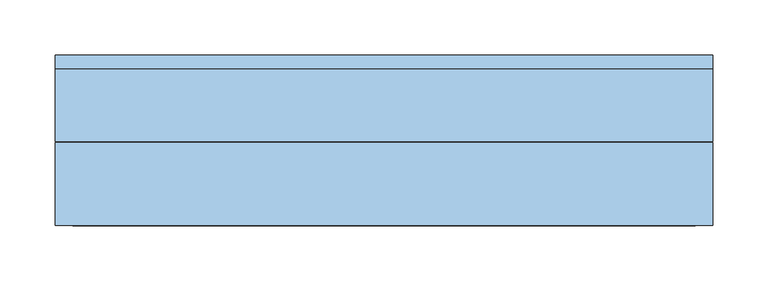
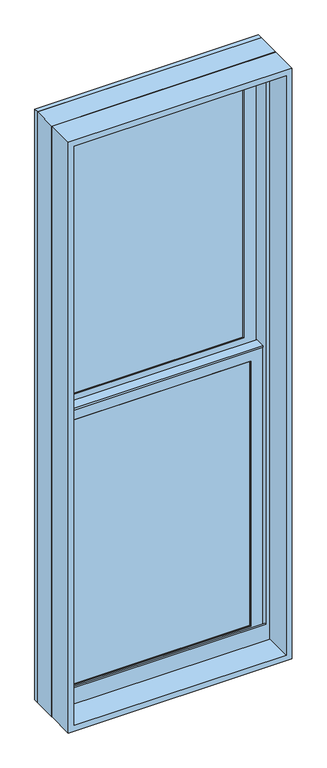
"""IFC4 building model written with IfcOpenShell, lengths in millimetres: window geometry, Window-Double_Hung-Marvin-Essential : ESDH2056."""

from ifc_helpers import new_model, si_unit, frame, origin, place, context, project, spatial, polyline, outline, extrude, faceted_brep, source, transform, mapped, element, save


def window_dac89900(model_context):
    return source(origin(), model_context, "Body", "SolidModel", [
        extrude(outline(polyline([(89.9583333, 20.6375), (89.9583333, 15.875), (70.9083333, 15.875), (70.9083333, 20.6375), (89.9583333, 20.6375)])), frame((0.0, 0.0, 831.85), z_axis=(0.0, 0.0, 1.0), x_axis=(1.0, 0.0, 0.0)), (0.0, 0.0, 1.0), 755.65),
        extrude(outline(polyline([(-70.9083333, 20.6375), (-70.9083333, 15.875), (-89.9583333, 15.875), (-89.9583333, 20.6375), (-70.9083333, 20.6375)])), frame((0.0, 0.0, 831.85), z_axis=(0.0, 0.0, 1.0), x_axis=(1.0, 0.0, 0.0)), (0.0, 0.0, 1.0), 755.65),
        extrude(outline(polyline([(241.3, 20.6375), (241.3, 15.875), (-241.3, 15.875), (-241.3, 20.6375), (241.3, 20.6375)])), frame((0.0, 0.0, 1200.15), z_axis=(0.0, 0.0, 1.0), x_axis=(1.0, 0.0, 0.0)), (0.0, 0.0, 1.0), 19.05),
        extrude(outline(polyline([(-89.9583333, 46.83125), (-89.9583333, 51.59375), (-70.9083333, 51.59375), (-70.9083333, 46.83125), (-89.9583333, 46.83125)])), frame((0.0, 0.0, 1625.6), z_axis=(0.0, 0.0, 1.0), x_axis=(1.0, 0.0, 0.0)), (0.0, 0.0, 1.0), 755.65),
        extrude(outline(polyline([(70.9083333, 46.83125), (70.9083333, 51.59375), (89.9583333, 51.59375), (89.9583333, 46.83125), (70.9083333, 46.83125)])), frame((0.0, 0.0, 1625.6), z_axis=(0.0, 0.0, 1.0), x_axis=(1.0, 0.0, 0.0)), (0.0, 0.0, 1.0), 755.65),
        extrude(outline(polyline([(-241.3, 46.83125), (-241.3, 51.59375), (241.3, 51.59375), (241.3, 46.83125), (-241.3, 46.83125)])), frame((0.0, 0.0, 1993.9), z_axis=(0.0, 0.0, 1.0), x_axis=(1.0, 0.0, 0.0)), (0.0, 0.0, 1.0), 19.05),
        extrude(outline(polyline([(89.9583333, 20.6375), (70.9083333, 20.6375), (70.9083333, 25.4), (89.9583333, 25.4), (89.9583333, 20.6375)])), frame((0.0, 0.0, 831.85), z_axis=(0.0, 0.0, 1.0), x_axis=(1.0, 0.0, 0.0)), (0.0, 0.0, 1.0), 755.65),
        extrude(outline(polyline([(-70.9083333, 20.6375), (-89.9583333, 20.6375), (-89.9583333, 25.4), (-70.9083333, 25.4), (-70.9083333, 20.6375)])), frame((0.0, 0.0, 831.85), z_axis=(0.0, 0.0, 1.0), x_axis=(1.0, 0.0, 0.0)), (0.0, 0.0, 1.0), 755.65),
        extrude(outline(polyline([(241.3, 20.6375), (-241.3, 20.6375), (-241.3, 25.4), (241.3, 25.4), (241.3, 20.6375)])), frame((0.0, 0.0, 1200.15), z_axis=(0.0, 0.0, 1.0), x_axis=(1.0, 0.0, 0.0)), (0.0, 0.0, 1.0), 19.05),
        extrude(outline(polyline([(-89.9583333, 56.35625), (-70.9083333, 56.35625), (-70.9083333, 51.59375), (-89.9583333, 51.59375), (-89.9583333, 56.35625)])), frame((0.0, 0.0, 1625.6), z_axis=(0.0, 0.0, 1.0), x_axis=(1.0, 0.0, 0.0)), (0.0, 0.0, 1.0), 755.65),
        extrude(outline(polyline([(70.9083333, 56.35625), (89.9583333, 56.35625), (89.9583333, 51.59375), (70.9083333, 51.59375), (70.9083333, 56.35625)])), frame((0.0, 0.0, 1625.6), z_axis=(0.0, 0.0, 1.0), x_axis=(1.0, 0.0, 0.0)), (0.0, 0.0, 1.0), 755.65),
        extrude(outline(polyline([(-241.3, 56.35625), (241.3, 56.35625), (241.3, 51.59375), (-241.3, 51.59375), (-241.3, 56.35625)])), frame((0.0, 0.0, 1993.9), z_axis=(0.0, 0.0, 1.0), x_axis=(1.0, 0.0, 0.0)), (0.0, 0.0, 1.0), 19.05),
        faceted_brep([(-268.2875, 5.6780605, 1617.5351748), (-268.2875, 5.6780605, 1612.9), (268.2875, 5.6780605, 1612.9), (268.2875, 5.6780605, 1617.5351748), (-268.2875, 34.8118605, 1617.5351748), (268.2875, 34.8118605, 1617.5351748), (268.2875, 34.8118605, 1612.9), (-268.2875, 34.8118605, 1612.9), (-268.2875, 30.1625, 1612.9), (-268.2875, 30.1625, 804.8625), (-268.2875, 8.9241104, 804.8625), (-268.2875, 8.9241104, 1612.9), (268.2875, 8.9241104, 1612.9), (268.2875, 30.1625, 1612.9), (268.2875, 8.9241104, 804.8625), (268.2875, 30.1625, 804.8625), (-252.4034752, 11.90625, 1598.6034752), (-252.4034752, 30.1625, 1598.6034752), (252.4034752, 30.1625, 1598.6034752), (252.4034752, 11.90625, 1598.6034752), (-235.74375, 10.4662439, 1581.94375), (-235.74375, 11.90625, 1581.94375), (235.74375, 11.90625, 1581.94375), (235.74375, 10.4662439, 1581.94375), (237.2858834, 8.9241104, 1583.4858834), (-237.2858834, 8.9241104, 1583.4858834), (252.4034752, 30.1625, 820.7465248), (252.4034752, 11.90625, 820.7465248), (235.74375, 11.90625, 837.40625), (235.74375, 10.4662439, 837.40625), (237.2858834, 8.9241104, 835.8641166), (-252.4034752, 30.1625, 820.7465248), (-252.4034752, 11.90625, 820.7465248), (-235.74375, 11.90625, 837.40625), (-235.74375, 10.4662439, 837.40625), (-237.2858834, 8.9241104, 835.8641166)], [[[0, 1, 2, 3]], [[4, 5, 6, 7]], [[1, 0, 4, 7, 8, 9, 10, 11]], [[2, 1, 11, 12]], [[7, 6, 13, 8]], [[3, 2, 12, 14, 15, 13, 6, 5]], [[0, 3, 5, 4]], [[16, 17, 18, 19]], [[20, 21, 22, 23]], [[20, 23, 24, 25]], [[19, 18, 26, 27]], [[23, 22, 28, 29]], [[24, 23, 29, 30]], [[27, 26, 31, 32]], [[29, 28, 33, 34]], [[30, 29, 34, 35]], [[15, 14, 10, 9]], [[15, 9, 8, 13], [18, 17, 31, 26]], [[17, 16, 32, 31]], [[16, 19, 27, 32], [22, 21, 33, 28]], [[21, 20, 34, 33]], [[20, 25, 35, 34]], [[10, 14, 12, 11], [25, 24, 30, 35]]]),
        extrude(outline(polyline([(38.5955581, 1598.6125), (33.5778968, 1598.6125), (33.5778968, 1600.2), (39.9405976, 1600.2), (39.9405976, 1598.6125), (61.515625, 1598.6125), (47.6307501, 1595.2975159), (38.5955581, 1595.2975159), (38.5955581, 1598.6125)])), frame((-268.2875, 0.0, 0.0), z_axis=(1.0, 0.0, 0.0), x_axis=(0.0, 1.0, 0.0)), (0.0, 0.0, 1.0), 536.575),
        faceted_brep([(298.45, 0.0, 774.7), (298.45, 0.0, 2438.4), (-298.45, 0.0, 2438.4), (-298.45, 0.0, 774.7), (272.25625, 0.0, 835.81875), (-272.25625, 0.0, 835.81875), (-272.25625, 0.0, 2412.20625), (272.25625, 0.0, 2412.20625), (272.25625, 3.96875, 774.7), (-272.25625, 3.96875, 774.7), (-272.25625, 3.96875, 835.81875), (272.25625, 3.96875, 835.81875), (-298.45, 65.6828125, 774.7), (-272.25625, 65.6828125, 774.7), (272.25625, 65.6828125, 774.7), (298.45, 65.6828125, 774.7), (-298.45, 65.6828125, 2438.4), (298.45, 65.6828125, 2438.4), (272.25625, 65.6828125, 2412.20625), (-272.25625, 65.6828125, 2412.20625)], [[[0, 1, 2, 3], [4, 5, 6, 7]], [[8, 9, 10, 11]], [[5, 4, 11, 10]], [[0, 3, 12, 13, 9, 8, 14, 15]], [[13, 12, 16, 17, 15, 14, 18, 19]], [[13, 19, 6, 5, 10, 9]], [[7, 6, 19, 18]], [[18, 14, 8, 11, 4, 7]], [[1, 0, 15, 17]], [[2, 1, 17, 16]], [[3, 2, 16, 12]]]),
        faceted_brep([(272.25625, 30.1625, 1606.55), (270.66875, 30.1625, 1606.55), (270.66875, 30.1625, 799.0544613), (272.25625, 30.1625, 799.0544613), (-270.66875, 30.1625, 1606.55), (-272.25625, 30.1625, 1606.55), (-272.25625, 30.1625, 799.0544613), (-270.66875, 30.1625, 799.0544613), (270.66875, 63.5, 1606.55), (272.25625, 63.5, 1606.55), (272.25625, 63.5, 792.5743077), (270.66875, 63.5, 792.5743077), (-272.25625, 63.5, 1606.55), (-270.66875, 63.5, 1606.55), (-270.66875, 63.5, 792.5743077), (-272.25625, 63.5, 792.5743077), (283.5108932, 3.96875, 804.1460105), (283.5108932, 3.96875, 774.7), (283.5108932, 65.6828125, 774.7), (283.5108932, 65.6828125, 792.150012), (-283.5108932, 3.96875, 774.7), (-283.5108932, 3.96875, 804.1460105), (-283.5108932, 65.6828125, 792.150012), (-283.5108932, 65.6828125, 774.7), (283.5108932, 78.58125, 789.6428097), (-283.5108932, 78.58125, 789.6428097), (-281.4971252, 68.2348864, 791.6539391), (-263.53135, 68.2348864, 791.6539391), (-263.53135, 65.6828125, 792.150012), (263.53135, 65.6828125, 792.150012), (263.53135, 68.2348864, 791.6539391), (281.4971252, 68.2348864, 791.6539391), (-298.45, 65.6828125, 774.7), (-298.45, 78.5948249, 774.7), (298.45, 78.5948249, 774.7), (298.45, 65.6828125, 774.7), (-298.45, 78.58125, 2438.4), (298.45, 78.58125, 2438.4), (283.5108932, 78.58125, 2423.4608932), (-283.5108932, 78.58125, 2423.4608932), (-298.45, 65.6828125, 2438.4), (-281.4971252, 68.2348864, 2421.4471252), (281.4971252, 68.2348864, 2421.4471252), (263.53135, 68.2348864, 2403.48135), (-263.53135, 68.2348864, 2403.48135), (-263.53135, 65.6828125, 2403.48135), (263.53135, 65.6828125, 2403.48135), (298.45, 65.6828125, 2438.4)], [[[0, 1, 2, 3]], [[4, 5, 6, 7]], [[8, 9, 10, 11]], [[12, 13, 14, 15]], [[1, 8, 11, 2]], [[9, 0, 3, 10]], [[1, 0, 9, 8]], [[5, 4, 13, 12]], [[5, 12, 15, 6]], [[13, 4, 7, 14]], [[16, 17, 18, 19]], [[20, 21, 22, 23]], [[24, 25, 26, 27, 28, 22, 21, 16, 19, 29, 30, 31], [3, 2, 11, 10], [7, 6, 15, 14]], [[17, 16, 21, 20]], [[17, 20, 23, 32, 33, 34, 35, 18]], [[34, 33, 36, 37], [25, 24, 38, 39]], [[33, 32, 40, 36]], [[39, 41, 26, 25]], [[41, 42, 31, 30, 43, 44, 27, 26]], [[44, 45, 28, 27]], [[40, 32, 23, 22, 28, 45, 46, 29, 19, 18, 35, 47]], [[36, 40, 47, 37]], [[39, 38, 42, 41]], [[44, 43, 46, 45]], [[34, 37, 47, 35]], [[42, 38, 24, 31]], [[46, 43, 30, 29]]]),
        extrude(outline(polyline([(248.44375, 11.90625), (-248.44375, 11.90625), (-248.44375, 15.08125), (248.44375, 15.08125), (248.44375, 11.90625)])), frame((0.0, 0.0, 824.70625), z_axis=(0.0, 0.0, 1.0), x_axis=(1.0, 0.0, 0.0)), (0.0, 0.0, 1.0), 769.9375),
        extrude(outline(polyline([(248.44375, 42.8625), (-248.44375, 42.8625), (-248.44375, 46.0375), (248.44375, 46.0375), (248.44375, 42.8625)])), frame((0.0, 0.0, 1618.45625), z_axis=(0.0, 0.0, 1.0), x_axis=(1.0, 0.0, 0.0)), (0.0, 0.0, 1.0), 769.9375),
        faceted_brep([(-235.74375, 31.194477, 1581.94375), (-237.2858834, 32.7366104, 1583.4858834), (237.2858834, 32.7366104, 1583.4858834), (235.74375, 31.194477, 1581.94375), (-235.74375, 30.1625, 1581.94375), (235.74375, 30.1625, 1581.94375), (-268.2875, 32.7366104, 1614.4875), (-268.2875, 30.1625, 1614.4875), (268.2875, 30.1625, 1614.4875), (268.2875, 32.7366104, 1614.4875), (237.2858834, 32.7366104, 835.8641166), (235.74375, 31.194477, 837.40625), (235.74375, 30.1625, 837.40625), (268.2875, 30.1625, 804.8625), (268.2875, 32.7366104, 804.8625), (-237.2858834, 32.7366104, 835.8641166), (-235.74375, 31.194477, 837.40625), (-235.74375, 30.1625, 837.40625), (-268.2875, 30.1625, 804.8625), (-268.2875, 32.7366104, 804.8625)], [[[0, 1, 2, 3]], [[4, 0, 3, 5]], [[6, 7, 8, 9]], [[3, 2, 10, 11]], [[5, 3, 11, 12]], [[9, 8, 13, 14]], [[11, 10, 15, 16]], [[12, 11, 16, 17]], [[14, 13, 18, 19]], [[9, 14, 19, 6], [1, 15, 10, 2]], [[16, 15, 1, 0]], [[17, 16, 0, 4]], [[7, 18, 13, 8], [5, 12, 17, 4]], [[19, 18, 7, 6]]]),
        faceted_brep([(-252.4034752, 42.8625, 2392.3534752), (-252.4034752, 61.11875, 2392.3534752), (252.4034752, 61.11875, 2392.3534752), (252.4034752, 42.8625, 2392.3534752), (-235.74375, 41.4224939, 2375.69375), (-235.74375, 42.8625, 2375.69375), (235.74375, 42.8625, 2375.69375), (235.74375, 41.4224939, 2375.69375), (-237.2858834, 39.8803604, 2377.2358834), (237.2858834, 39.8803604, 2377.2358834), (-268.2875, 61.11875, 2408.2375), (-268.2875, 39.8803604, 2408.2375), (268.2875, 39.8803604, 2408.2375), (268.2875, 61.11875, 2408.2375), (252.4034752, 61.11875, 1614.4965248), (252.4034752, 42.8625, 1614.4965248), (235.74375, 42.8625, 1631.15625), (235.74375, 41.4224939, 1631.15625), (237.2858834, 39.8803604, 1629.6141166), (268.2875, 39.8803604, 1598.6125), (268.2875, 61.11875, 1598.6125), (-252.4034752, 61.11875, 1614.4965248), (-252.4034752, 42.8625, 1614.4965248), (-235.74375, 42.8625, 1631.15625), (-235.74375, 41.4224939, 1631.15625), (-237.2858834, 39.8803604, 1629.6141166), (-268.2875, 39.8803604, 1598.6125), (-268.2875, 61.11875, 1598.6125)], [[[0, 1, 2, 3]], [[4, 5, 6, 7]], [[8, 4, 7, 9]], [[10, 11, 12, 13]], [[3, 2, 14, 15]], [[7, 6, 16, 17]], [[9, 7, 17, 18]], [[13, 12, 19, 20]], [[15, 14, 21, 22]], [[17, 16, 23, 24]], [[18, 17, 24, 25]], [[20, 19, 26, 27]], [[13, 20, 27, 10], [1, 21, 14, 2]], [[22, 21, 1, 0]], [[3, 15, 22, 0], [5, 23, 16, 6]], [[24, 23, 5, 4]], [[25, 24, 4, 8]], [[11, 26, 19, 12], [9, 18, 25, 8]], [[27, 26, 11, 10]]]),
        faceted_brep([(-268.2875, 61.11875, 1598.6125), (-268.2875, 63.6928604, 1598.6125), (268.2875, 63.6928604, 1598.6125), (268.2875, 61.11875, 1598.6125), (-235.74375, 62.150727, 1631.15625), (-235.74375, 61.11875, 1631.15625), (235.74375, 61.11875, 1631.15625), (235.74375, 62.150727, 1631.15625), (-237.2858834, 63.6928604, 1629.6141166), (237.2858834, 63.6928604, 1629.6141166), (268.2875, 63.6928604, 2408.2375), (268.2875, 61.11875, 2408.2375), (235.74375, 61.11875, 2375.69375), (235.74375, 62.150727, 2375.69375), (237.2858834, 63.6928604, 2377.2358834), (-268.2875, 63.6928604, 2408.2375), (-268.2875, 61.11875, 2408.2375), (-235.74375, 61.11875, 2375.69375), (-235.74375, 62.150727, 2375.69375), (-237.2858834, 63.6928604, 2377.2358834)], [[[0, 1, 2, 3]], [[4, 5, 6, 7]], [[8, 4, 7, 9]], [[3, 2, 10, 11]], [[7, 6, 12, 13]], [[9, 7, 13, 14]], [[11, 10, 15, 16]], [[13, 12, 17, 18]], [[14, 13, 18, 19]], [[16, 15, 1, 0]], [[3, 11, 16, 0], [5, 17, 12, 6]], [[18, 17, 5, 4]], [[19, 18, 4, 8]], [[1, 15, 10, 2], [9, 14, 19, 8]]]),
        extrude(outline(polyline([(248.44375, 26.19375), (-248.44375, 26.19375), (-248.44375, 30.1625), (248.44375, 30.1625), (248.44375, 26.19375)])), frame((0.0, 0.0, 824.70625), z_axis=(0.0, 0.0, 1.0), x_axis=(1.0, 0.0, 0.0)), (0.0, 0.0, 1.0), 769.9375),
        extrude(outline(polyline([(248.44375, 57.15), (-248.44375, 57.15), (-248.44375, 61.11875), (248.44375, 61.11875), (248.44375, 57.15)])), frame((0.0, 0.0, 1618.45625), z_axis=(0.0, 0.0, 1.0), x_axis=(1.0, 0.0, 0.0)), (0.0, 0.0, 1.0), 769.9375),
        extrude(outline(polyline([(2438.4, 298.45), (2438.4, -298.45), (774.7, -298.45), (774.7, 298.45), (2438.4, 298.45)]), holes=[polyline([(2422.525, 282.575), (790.575, 282.575), (790.575, -282.575), (2422.525, -282.575), (2422.525, 282.575)])]), frame((0.0, -76.2, 0.0), z_axis=(0.0, 1.0, 0.0), x_axis=(0.0, 0.0, 1.0)), (0.0, 0.0, 1.0), 75.40625),
    ])


if __name__ == "__main__":
    model = new_model("IFC4")
    model_context = context("Model", 3, world=origin())
    ifc_project = project(units=[si_unit("LENGTHUNIT", "METRE", prefix="MILLI")], contexts=[model_context])
    site = spatial("IfcSite", under=ifc_project)
    building = spatial("IfcBuilding", under=site)
    placement = place(None, origin())
    window_shape = window_dac89900(model_context)
    element("IfcWindow", 1, ObjectType="Window-Double_Hung-Marvin-Essential : ESDH2056", at=placement, inside=building, context=model_context, shape_type="MappedRepresentation", body=[
        mapped(window_shape, transform((0.0, 0.0, 0.0), x_axis=(1.0, 0.0, 0.0), y_axis=(0.0, 1.0, 0.0), z_axis=(0.0, 0.0, 1.0))),
    ])
    save(model, "model.ifc")

# Revit data of these elements
# Type "Window-Double_Hung-Marvin-Essential : ESDH2056"
#   Type Mark = "69"
#   Window Type = "Essential Double Hung"
#   Product data url = "https://bimobject.com/marvin-windows-and-doors/product/marvin-dhwau"
#   Product Guid = "c4a96547-874c-4385-91dc-a058adc19d98"
#   Frame = "All Ultrex"
#   Egress Window = "No"
#   URL = "www.marvin.com"
#   Model = "ESDH2056"
#   Manufacturer = "Marvin Windows and Doors"
#   Label Egress = ""
#   Glass Type = "IG Low E II with Argon"
#   Design Pressure = "DP40"
#   Description = "2466 DBHG"
#   Analytic Construction = "<None>"
#   Prairie Corner Width = 0' - 4"
#   Prairie Corner Height = 0' - 4"
#   Egress Width = 1' - 8 9/16"
#   Egress Height = 2' - 4 27/128"
#   Rough Width = 2' - 0"
#   Rough Height = 5' - 6"
#   Nominal Width = 2' - 0"
#   Nominal Height = 5' - 6"
#   Inset to Installation Flange [instance default] = 0' - 1"
#   Height = 5' - 5 1/2"
#   Egress Area = 4.02838 SF
#   Default Head Height = 8' - 0"
#   Width = 1' - 11 1/2"
#   Daylight Area = 7.55713 SF
#   DLO Width = 1' - 6 9/16"
#   DLO Height = 2' - 5 5/16"
#   Muntins Top Sash = yes
#   Lites Wide Top Sash = 3
#   Lites Wide Bottom Sash = 3
#   Lites High Top Sash = 2
#   Lites High Bottom Sash = 2
#   Lite Cut Prairie 9 = no
#   Lite Cut HV Grid = yes
#   Muntins Bottom Sash = yes
#   Label Visibility = no
#   Jamb Extension Visibility = yes
#   Edition number = 1
#   Interior Material = Ultrex-Marvin-Stonewhite
#   Glazing Material = Glass-Marvin-IG Low E II with Argon
#   Cladding Material = Ultrex-Marvin-Pebblegray
#   Wall Closure = (empty or 0)
#   Assembly Code = ""
# Element 1 (IfcWindow, "Window-Double_Hung-Marvin-Essential : ESDH2056")
#   Materials on its faces: "Ultrex-Marvin-Pebblegray", "Ultrex-Marvin-Stonewhite", "Glass-Marvin-IG Low E II with Argon"
# Materials
#   "Ultrex-Marvin-Stonewhite": class "Paint", colour RGB 250 251 245, transparency 0
#   "Glass-Marvin-IG Low E II with Argon": class "Glass", colour RGB 0 128 192, transparency 0.85
#   "Ultrex-Marvin-Pebblegray": class "Paint", colour RGB 189 185 173, transparency 0
